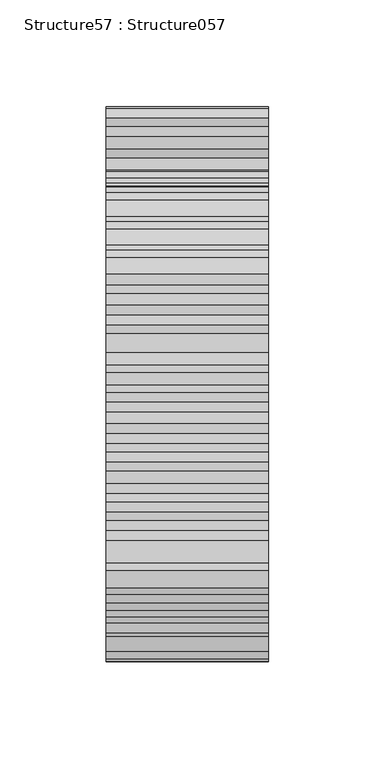
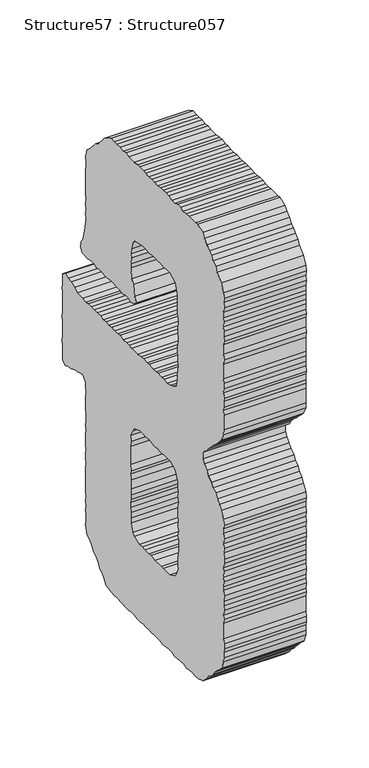
"""IFC4 building model written with IfcOpenShell, lengths in millimetres: proxy geometry, Structure57 : Structure057."""

from ifc_helpers import new_model, si_unit, frame, origin, place, context, project, spatial, polyline, outline, extrude, source, transform, mapped, element, save


def structure57_structure057_54d458d5(model_context):
    return source(origin(), model_context, "Body", "SweptSolid", [
        extrude(outline(polyline([(257601.6917186, 3904.3901392), (257600.5107297, 3908.46423), (257601.089992, 3912.5896682), (257601.089992, 3917.8479571), (257601.6917186, 3921.9733953), (257601.089992, 3927.2332888), (257601.6917186, 3930.7329312), (257601.6917186, 3936.0345445), (257600.5107297, 3941.2912288), (257601.089992, 3945.9766739), (257600.5107297, 3950.6765605), (257601.6917186, 3955.360401), (257605.2122209, 3962.9774586), (257612.2323656, 3968.8198235), (257613.9942213, 3973.5197101), (257618.673248, 3976.4368811), (257621.5936282, 3979.9621971), (257624.5348682, 3982.3225704), (257628.0553705, 3986.4046842), (257632.1567396, 3989.9460463), (257635.0979796, 3994.0233463), (257643.2991132, 3996.9645864), (257646.7987556, 3996.390138), (257657.361867, 3996.390138), (257662.0424983, 3995.7803883), (257666.7231296, 3995.7803883), (257670.8228941, 3996.9645864), (257675.5035254, 3996.9645864), (257679.6257544, 3995.7803883), (257684.3063857, 3995.7803883), (257690.1455415, 3996.390138), (257694.2677704, 3996.9645864), (257698.9484017, 3996.390138), (257703.0706307, 3996.390138), (257707.751262, 3995.7803883), (257712.4318933, 3996.390138), (257717.7126467, 3995.7803883), (257722.393278, 3995.7803883), (257727.0739093, 3996.390138), (257730.5944116, 3996.390138), (257736.4560318, 3996.9645864), (257739.9765341, 3996.9645864), (257745.8381543, 3995.7803883), (257754.6185501, 3995.7803883), (257758.7199192, 3996.9645864), (257763.423015, 3995.7803883), (257768.1020417, 3996.9645864), (257773.3619352, 3996.390138), (257777.4633043, 3996.390138), (257782.7440577, 3996.9645864), (257790.3659291, 3992.8375436), (257793.8655715, 3989.9460463), (257796.2050848, 3986.4046842), (257803.8269562, 3978.8036727), (257807.349063, 3976.4368811), (257809.6885764, 3973.5197101), (257817.3104478, 3965.3201811), (257820.83095, 3962.3757319), (257823.172068, 3954.1778075), (257822.5928058, 3950.0940891), (257822.5928058, 3945.9766739), (257823.172068, 3940.718385), (257823.172068, 3935.4328178), (257823.7737947, 3930.7329312), (257823.7737947, 3921.3748778), (257823.172068, 3917.8479571), (257822.5928058, 3913.1641166), (257823.172068, 3908.46423), (257822.5928058, 3902.6314927), (257823.7737947, 3898.5301236), (257822.5928058, 3893.246161), (257823.172068, 3889.1463965), (257825.5115813, 3880.3627915), (257827.8510947, 3870.9790644), (257830.7939393, 3866.3032469), (257831.3507371, 3861.0192843), (257829.0320836, 3856.3161885), (257825.5115813, 3856.3161885), (257820.2292233, 3855.7353217), (257814.9709344, 3856.9179152), (257810.2678386, 3856.9179152), (257806.188934, 3855.7353217), (257800.9081806, 3856.9179152), (257796.8068115, 3856.9179152), (257792.1261802, 3855.7353217), (257782.7440577, 3856.9179152), (257778.6442932, 3856.9179152), (257773.9411974, 3856.3161885), (257768.6813039, 3856.9179152), (257763.423015, 3855.7353217), (257759.2991814, 3856.9179152), (257755.1994169, 3856.9179152), (257750.5187856, 3855.7353217), (257745.8381543, 3856.9179152), (257741.7159254, 3860.4432313), (257744.6571654, 3865.1190488), (257746.4174165, 3875.686974), (257749.3377967, 3879.1769888), (257750.5187856, 3889.1463965), (257750.5187856, 3893.246161), (257749.3377967, 3899.7046941), (257750.5187856, 3903.2059411), (257749.9170589, 3908.46423), (257746.9966788, 3916.6653636), (257744.6571654, 3919.6066036), (257735.8543051, 3921.3748778), (257731.7754005, 3922.5494483), (257726.4721826, 3921.9733953), (257721.2122891, 3921.3748778), (257717.7126467, 3921.9733953), (257711.8301666, 3922.5494483), (257707.1495353, 3921.9733953), (257703.0706307, 3922.5494483), (257697.7674128, 3921.3748778), (257692.5075193, 3922.5494483), (257687.826888, 3922.5494483), (257679.0240277, 3917.8479571), (257675.5035254, 3908.46423), (257675.5035254, 3890.905043), (257674.345001, 3885.0626781), (257674.345001, 3880.9452629), (257674.9242632, 3876.263027), (257674.9242632, 3871.5599312), (257674.345001, 3866.8776953), (257674.345001, 3862.8036045), (257675.5035254, 3856.9179152), (257675.5035254, 3852.8181507), (257674.9242632, 3848.7167816), (257674.9242632, 3843.432819), (257674.345001, 3839.3587282), (257675.5035254, 3829.9733965), (257675.5035254, 3824.1149855), (257677.2637766, 3818.2309008), (257681.3651457, 3815.3313805), (257687.2476258, 3812.3901405), (257692.5075193, 3811.2043377), (257697.1881506, 3812.3901405), (257701.2879151, 3811.7884138), (257707.1495353, 3812.3901405), (257710.6716422, 3811.7884138), (257715.3506689, 3811.2043377), (257721.2122891, 3812.3901405), (257724.7327914, 3811.7884138), (257730.0151494, 3812.3901405), (257734.6957807, 3811.7884138), (257739.9765341, 3811.2043377), (257749.3377967, 3811.2043377), (257753.4375612, 3811.7884138), (257757.5389303, 3811.7884138), (257763.423015, 3811.2043377), (257768.1020417, 3812.3901405), (257772.1809463, 3811.7884138), (257776.8824375, 3811.7884138), (257781.5630688, 3812.3901405), (257786.8229623, 3811.2043377), (257790.9451913, 3811.7884138), (257795.0465604, 3811.2043377), (257799.7271917, 3812.3901405), (257805.0079451, 3812.3901405), (257810.2678386, 3811.7884138), (257814.3900676, 3812.3901405), (257819.6499611, 3812.3901405), (257823.7737947, 3811.2043377), (257828.4528214, 3812.3901405), (257837.2348218, 3812.3901405), (257841.3345863, 3815.3313805), (257847.173742, 3817.090027), (257851.8768378, 3817.6741031), (257855.9766023, 3820.015221), (257860.0779714, 3817.090027), (257860.0779714, 3806.5317294), (257861.2364958, 3803.0064134), (257860.6796981, 3798.3305959), (257860.0779714, 3792.4705802), (257860.6796981, 3788.3611881), (257860.0779714, 3783.0868532), (257860.6796981, 3779.5872107), (257861.2364958, 3774.8857196), (257860.0779714, 3770.2018791), (257860.0779714, 3760.818152), (257860.6796981, 3755.559863), (257861.2364958, 3751.4424479), (257860.0779714, 3745.6000829), (257860.0779714, 3732.1149867), (257855.9766023, 3729.1737467), (257851.295971, 3731.5325153), (257846.5944798, 3732.1149867), (257841.3345863, 3734.47536), (257836.6539549, 3735.0578314), (257828.4528214, 3737.9750024), (257823.172068, 3733.2991849), (257823.172068, 3728.5992983), (257822.5928058, 3723.9154578), (257823.172068, 3718.0554422), (257823.172068, 3713.9556777), (257823.7737947, 3708.6717151), (257822.5928058, 3700.4705815), (257822.5928058, 3695.786741), (257823.7737947, 3690.512406), (257822.5928058, 3686.4030139), (257823.172068, 3682.3289231), (257823.7737947, 3676.4432338), (257823.172068, 3672.3691429), (257822.5928058, 3667.0851803), (257823.7737947, 3663.5598643), (257823.172068, 3658.8840468), (257822.5928058, 3653.6000842), (257823.7737947, 3649.5003197), (257823.172068, 3644.2420307), (257823.172068, 3636.0408972), (257823.7737947, 3631.3410106), (257823.7737947, 3626.0554434), (257822.5928058, 3621.3732075), (257823.7737947, 3617.2718384), (257822.5928058, 3612.5976255), (257823.172068, 3607.8961343), (257822.5928058, 3602.6298224), (257822.5928058, 3598.5284533), (257823.7737947, 3593.2541183), (257820.83095, 3585.0706354), (257817.3104478, 3582.7102621), (257813.2090787, 3578.6104977), (257810.8695653, 3574.5107332), (257806.188934, 3571.5678885), (257803.247694, 3569.2524442), (257800.9081806, 3564.54293), (257796.2050848, 3561.025637), (257793.8655715, 3558.684519), (257790.3659291, 3554.0087015), (257782.142331, 3552.242032), (257778.065031, 3551.6675836), (257772.782673, 3552.242032), (257764.559075, 3552.242032), (257759.2991814, 3551.0658569), (257754.6185501, 3551.0658569), (257749.9170589, 3552.242032), (257745.8381543, 3552.242032), (257741.1591276, 3551.0658569), (257735.2750429, 3551.0658569), (257731.1736738, 3552.242032), (257726.4721826, 3551.6675836), (257721.2122891, 3552.242032), (257717.7126467, 3551.6675836), (257712.4318933, 3552.242032), (257703.6514975, 3552.242032), (257699.527664, 3551.0658569), (257693.6885082, 3551.6675836), (257689.5662792, 3552.242032), (257684.8856479, 3552.242032), (257680.8067433, 3551.0658569), (257671.4246208, 3552.242032), (257665.5630006, 3552.242032), (257661.4407716, 3551.0658569), (257656.1808781, 3552.242032), (257652.6603758, 3552.242032), (257646.7987556, 3551.6675836), (257642.1181243, 3552.242032), (257635.0979796, 3554.5831499), (257631.5774774, 3557.5003209), (257627.4761083, 3561.6257591), (257625.7158572, 3564.54293), (257621.0352258, 3568.0682461), (257618.673248, 3570.9854171), (257614.5734835, 3575.6853037), (257612.2323656, 3578.0103756), (257607.5308744, 3582.7102621), (257604.6329587, 3585.0706354), (257601.6917186, 3593.2541183), (257601.089992, 3597.9540049), (257601.089992, 3603.2122938), (257600.5107297, 3606.7295868), (257600.5107297, 3612.0135494), (257601.6917186, 3616.0972679), (257601.6917186, 3631.3410106), (257600.5107297, 3636.0408972), (257601.6917186, 3638.9580681), (257600.5107297, 3644.8245022), (257601.089992, 3648.9258713), (257601.089992, 3652.9999621), (257600.5107297, 3658.8840468), (257601.6917186, 3663.5598643), (257601.6917186, 3667.0851803), (257601.089992, 3672.3691429), (257601.6917186, 3676.4432338), (257601.089992, 3682.3289231), (257601.6917186, 3685.8285655), (257600.5107297, 3690.512406), (257600.5107297, 3694.6298211), (257601.089992, 3700.4705815), (257600.5107297, 3705.1720727), (257601.6917186, 3709.2718371), (257600.5107297, 3714.5301261), (257601.6917186, 3719.2316172), (257601.6917186, 3723.9154578), (257600.5107297, 3728.0152223), (257601.6917186, 3733.2991849), (257605.2122209, 3739.7416719), (257608.1326011, 3743.8414364), (257611.6531034, 3747.3587295), (257613.9942213, 3751.4424479), (257618.673248, 3753.8012165), (257621.0352258, 3757.8753073), (257625.7158572, 3761.418274), (257628.6570972, 3764.9435901), (257632.1567396, 3769.0176809), (257634.496253, 3772.5606477), (257634.496253, 3779.0031347), (257632.1567396, 3781.3282066), (257628.0553705, 3784.2614236), (257625.7158572, 3787.7867397), (257622.1953549, 3791.8865042), (257615.1527458, 3798.3305959), (257611.0738411, 3802.448011), (257608.7118633, 3804.7730829), (257605.2122209, 3808.290376), (257601.6917186, 3815.9154565), (257601.089992, 3821.1737455), (257601.089992, 3835.2332901), (257601.6917186, 3839.9331766), (257601.089992, 3843.432819), (257601.089992, 3849.3008577), (257600.5107297, 3852.2340747), (257601.6917186, 3856.9179152), (257601.089992, 3861.6178018), (257601.089992, 3866.8776953), (257601.6917186, 3870.9790644), (257601.6917186, 3885.0626781), (257600.5107297, 3890.320967), (257601.6917186, 3895.0048075), (257601.6917186, 3904.3901392)]), holes=[polyline([(257744.6571654, 3735.0578314), (257736.4560318, 3737.9750024), (257731.1736738, 3737.9750024), (257727.6531716, 3737.400554), (257721.7915513, 3737.9750024), (257716.5316578, 3737.400554), (257712.4318933, 3736.7988273), (257707.751262, 3737.9750024), (257703.0706307, 3736.7988273), (257697.1881506, 3737.9750024), (257693.6885082, 3737.400554), (257687.826888, 3737.9750024), (257679.6257544, 3733.8736333), (257675.5035254, 3725.0996559), (257675.5035254, 3719.2316172), (257674.9242632, 3715.1302482), (257675.5035254, 3710.4560353), (257674.345001, 3705.1720727), (257675.5035254, 3700.4705815), (257675.5035254, 3691.6869765), (257674.9242632, 3687.0127636), (257675.5035254, 3681.7271964), (257674.345001, 3677.6274319), (257675.5035254, 3672.3691429), (257674.345001, 3668.8261762), (257674.345001, 3658.8840468), (257675.5035254, 3649.5003197), (257675.5035254, 3644.2420307), (257674.9242632, 3639.5405396), (257678.4447655, 3632.5155811), (257680.2050166, 3630.1824862), (257687.826888, 3626.6571701), (257698.3691395, 3626.6571701), (257701.8896418, 3626.0554434), (257711.8301666, 3626.0554434), (257717.7126467, 3627.2396415), (257721.7915513, 3626.6571701), (257727.6531716, 3626.6571701), (257731.7754005, 3627.2396415), (257736.4560318, 3626.6571701), (257744.6571654, 3629.5984101), (257747.5984054, 3631.915459), (257749.3377967, 3640.114988), (257749.9170589, 3644.8245022), (257749.9170589, 3650.1004418), (257750.5187856, 3654.7842823), (257750.5187856, 3659.4584952), (257749.9170589, 3662.9854159), (257749.3377967, 3667.6853024), (257749.9170589, 3672.9435914), (257749.9170589, 3681.7271964), (257750.5187856, 3687.587212), (257749.3377967, 3691.0868544), (257750.5187856, 3696.9709391), (257750.5187856, 3714.5301261), (257749.3377967, 3719.8140887), (257750.5187856, 3725.0996559), (257746.9966788, 3731.5325153), (257744.6571654, 3735.0578314)])]), frame((-38594.2176606, 0.0, 0.0), z_axis=(1.0, 0.0, 0.0), x_axis=(0.0, 1.0, 0.0)), (0.0, 0.0, 1.0), 76.2),
    ])


if __name__ == "__main__":
    model = new_model("IFC4")
    model_context = context("Model", 3, world=origin())
    ifc_project = project(units=[si_unit("LENGTHUNIT", "METRE", prefix="MILLI")], contexts=[model_context])
    site = spatial("IfcSite", under=ifc_project)
    building = spatial("IfcBuilding", under=site)
    placement = place(None, origin())
    structure57_structure057_shape = structure57_structure057_54d458d5(model_context)
    element("IfcBuildingElementProxy", 1, Name="Structure57 : Structure057", ObjectType="Structure57 : Structure057", at=placement, inside=building, context=model_context, shape_type="MappedRepresentation", body=[
        mapped(structure57_structure057_shape, transform((0.0, 0.0, 0.0), x_axis=(1.0, 0.0, 0.0), y_axis=(0.0, 1.0, 0.0), z_axis=(0.0, 0.0, 1.0))),
    ])
    save(model, "model.ifc")

# Revit data of these elements
# Type "Structure57 : Structure057"
#   NameOverride = "Structure057"
# Element 1 (IfcBuildingElementProxy, "Structure57 : Structure057")
#   Materials on its faces: "BRUSHED ALUM. LETTERING"
# Materials
#   "BRUSHED ALUM. LETTERING": class "Unassigned", colour RGB 169 181 186, transparency 0, Cost = 0
